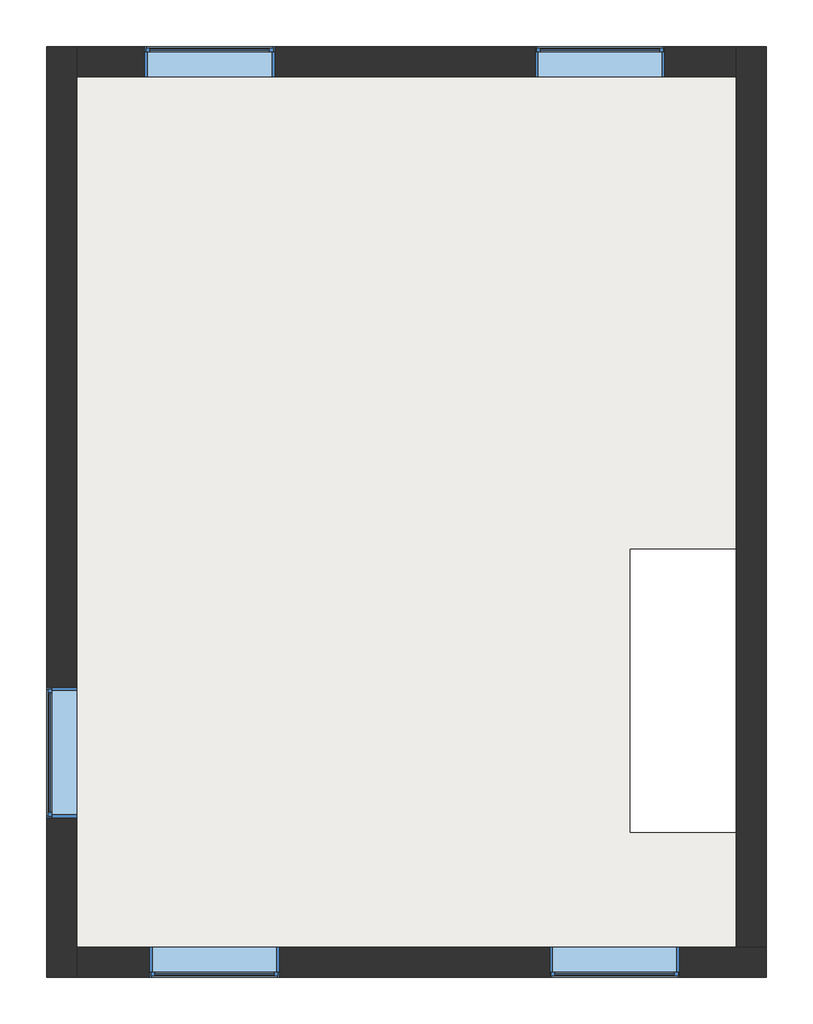
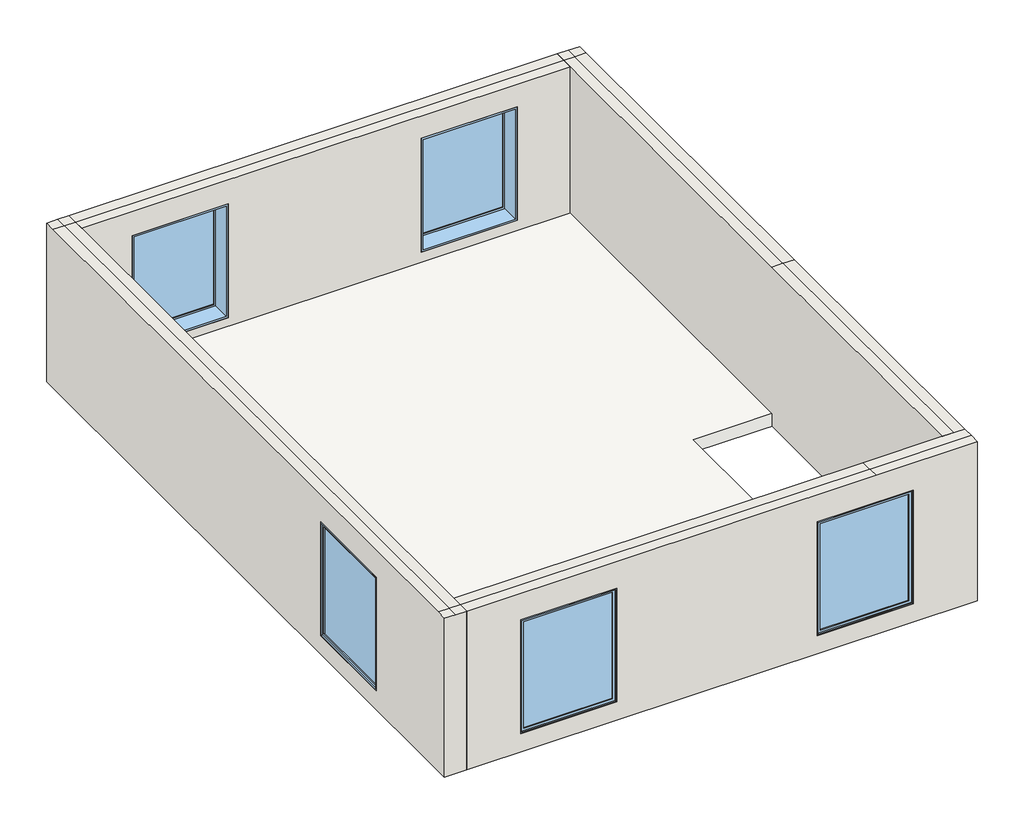
# One storey: 5 windows, 4 walls, 1 slab.
"""IFC4 building model written with IfcOpenShell, lengths in millimetres."""

import ifcopenshell
import ifcopenshell.guid

model = None  # the IFC model being written
_history = None  # IfcOwnerHistory: only IFC2X3 demands one
_inside = {}  # id of a spatial element -> (the spatial element, [elements in it])
_under = {}  # id of a project, library or spatial element -> (it, [spatial elements below it])
_declared = {}  # id of a project -> (the project, [libraries it declares])
_typed = {}  # id of a type object -> (the type object, [elements of that type])
_made_of = {}  # id of a material, layer set ... -> (it, [elements and type objects made of it])


def new_model(schema):
    """Start an empty IFC model of exactly this schema.

    Asked for "IFC4X3", IfcOpenShell would pick the latest addendum, in which some entities
    have other attributes; the version numbers below select the first issue.
    IFC2X3 requires an IfcOwnerHistory on every rooted entity: one is made here for all.
    """
    global model, _history
    if schema == "IFC4X3":
        model = ifcopenshell.file(schema_version=(4, 3, 0, 0))
    else:
        model = ifcopenshell.file(schema=schema)
    _inside.clear()
    _under.clear()
    _declared.clear()
    _typed.clear()
    _made_of.clear()
    _history = None
    if model.schema == "IFC2X3":
        org = make("IfcOrganization", Name="unknown")
        user = make(
            "IfcPersonAndOrganization",
            ThePerson=make("IfcPerson", FamilyName="unknown"),
            TheOrganization=org,
        )
        app = make(
            "IfcApplication",
            ApplicationDeveloper=org,
            Version="unknown",
            ApplicationFullName="unknown",
            ApplicationIdentifier="unknown",
        )
        _history = make(
            "IfcOwnerHistory",
            OwningUser=user,
            OwningApplication=app,
            ChangeAction="ADDED",
            CreationDate=0,
        )
    return model


def make(cls, **values):
    """One entity of the class cls with the attributes given. An attribute that is None is left unset."""
    return model.create_entity(
        cls, **{name: value for name, value in values.items() if value is not None}
    )


def rooted(cls, **values):
    """An entity with a GlobalId (a new one), such as an element, a storey or a relation."""
    return make(cls, GlobalId=ifcopenshell.guid.new(), OwnerHistory=_history, **values)


def si_unit(unit_type, name, prefix=None):
    """IfcSIUnit, for example si_unit("LENGTHUNIT", "METRE", prefix="MILLI")."""
    return make("IfcSIUnit", UnitType=unit_type, Prefix=prefix, Name=name)


def assignment(units):
    """IfcUnitAssignment: the units of a project."""
    return None if units is None else make("IfcUnitAssignment", Units=units)


def point(xyz):
    """IfcCartesianPoint."""
    return None if xyz is None else make("IfcCartesianPoint", Coordinates=xyz)


def direction(xyz):
    """IfcDirection."""
    return None if xyz is None else make("IfcDirection", DirectionRatios=xyz)


def frame(location, z_axis=None, x_axis=None):
    """IfcAxis2Placement3D, a coordinate frame: its origin and axes. An axis left out is left unset."""
    return make(
        "IfcAxis2Placement3D",
        Location=point(location),
        Axis=direction(z_axis),
        RefDirection=direction(x_axis),
    )


def origin():
    """The frame at (0, 0, 0) with its axes left unset."""
    return frame((0.0, 0.0, 0.0))


def place(relative_to, where):
    """IfcLocalPlacement: puts the frame where relative to a parent placement (None: the world)."""
    return make(
        "IfcLocalPlacement", PlacementRelTo=relative_to, RelativePlacement=where
    )


def context(
    kind, dimensions, precision=None, world=None, true_north=None, identifier=None
):
    """IfcGeometricRepresentationContext, for example the 3D "Model" context."""
    return make(
        "IfcGeometricRepresentationContext",
        ContextIdentifier=identifier,
        ContextType=kind,
        CoordinateSpaceDimension=dimensions,
        Precision=precision,
        WorldCoordinateSystem=world,
        TrueNorth=true_north,
    )


def project(units=None, contexts=None):
    """IfcProject with its units and contexts."""
    return rooted(
        "IfcProject",
        Name="project",
        RepresentationContexts=contexts,
        UnitsInContext=assignment(units),
    )


def spatial(cls, under=None, at=None, **own):
    """A site, building, storey or space (cls), placed at a placement, below another one or the project."""
    s = rooted(cls, ObjectPlacement=at, **own)
    if under is not None:
        _under.setdefault(under.id(), (under, []))[1].append(s)
    return s


def polyline(points):
    """IfcPolyline through the points."""
    return make("IfcPolyline", Points=[point(p) for p in points])


def outline(outer, holes=None, kind="AREA"):
    """IfcArbitraryClosedProfileDef: a profile drawn as a closed curve; with holes, ...WithVoids."""
    if holes is None:
        return make("IfcArbitraryClosedProfileDef", ProfileType=kind, OuterCurve=outer)
    return make(
        "IfcArbitraryProfileDefWithVoids",
        ProfileType=kind,
        OuterCurve=outer,
        InnerCurves=holes,
    )


def extrude(swept, where, along, depth):
    """IfcExtrudedAreaSolid: the profile swept, set in the frame where, extruded along a direction by depth."""
    return make(
        "IfcExtrudedAreaSolid",
        SweptArea=swept,
        Position=where,
        ExtrudedDirection=direction(along),
        Depth=depth,
    )


def faces_of(points, faces, orient=None, outer=None):
    """IfcFace entities. A face is a list of loops; a loop is a list of indices into points, from 0.

    orient and outer hold one flag for each loop. By default every Orientation is true, the
    first loop of a face is its IfcFaceOuterBound and the others are IfcFaceBound.
    """
    made = []
    for i, loops in enumerate(faces):
        bounds = []
        for j, loop in enumerate(loops):
            is_outer = j == 0 if outer is None else outer[i][j]
            bounds.append(
                make(
                    "IfcFaceOuterBound" if is_outer else "IfcFaceBound",
                    Bound=make("IfcPolyLoop", Polygon=[points[k] for k in loop]),
                    Orientation=True if orient is None else orient[i][j],
                )
            )
        made.append(make("IfcFace", Bounds=bounds))
    return made


def faceted_brep(points, faces, orient=None, outer=None, voids=None):
    """IfcFacetedBrep: a solid bounded by flat faces; with voids (closed shells), ...WithVoids."""
    shared = [point(p) for p in points]
    hull = make("IfcClosedShell", CfsFaces=faces_of(shared, faces, orient, outer))
    if voids is None:
        return make("IfcFacetedBrep", Outer=hull)
    return make(
        "IfcFacetedBrepWithVoids",
        Outer=hull,
        Voids=[
            make(cls, CfsFaces=faces_of(shared, fs, o, b)) for cls, fs, o, b in voids
        ],
    )


def shape(context_of_items, identifier, shape_type, items):
    """IfcShapeRepresentation: the items that make up one representation, for example the "Body"."""
    return make(
        "IfcShapeRepresentation",
        ContextOfItems=context_of_items,
        RepresentationIdentifier=identifier,
        RepresentationType=shape_type,
        Items=items,
    )


def source(mapping_origin, context_of_items, identifier, shape_type, items):
    """IfcRepresentationMap: a shape defined once, which mapped items show again and again."""
    return make(
        "IfcRepresentationMap",
        MappingOrigin=mapping_origin,
        MappedRepresentation=shape(context_of_items, identifier, shape_type, items),
    )


def transform(
    local_origin,
    x_axis=None,
    y_axis=None,
    z_axis=None,
    scale=None,
    scale2=None,
    scale3=None,
    uniform=True,
):
    """IfcCartesianTransformationOperator3D, or its non-uniform kind. x_axis, y_axis, z_axis: its Axis1, 2, 3."""
    if uniform:
        return make(
            "IfcCartesianTransformationOperator3D",
            Axis1=direction(x_axis),
            Axis2=direction(y_axis),
            LocalOrigin=point(local_origin),
            Scale=scale,
            Axis3=direction(z_axis),
        )
    return make(
        "IfcCartesianTransformationOperator3DnonUniform",
        Axis1=direction(x_axis),
        Axis2=direction(y_axis),
        LocalOrigin=point(local_origin),
        Scale=scale,
        Axis3=direction(z_axis),
        Scale2=scale2,
        Scale3=scale3,
    )


def mapped(mapping_source, mapping_target):
    """IfcMappedItem: shows the shape of a source again, moved by a transform."""
    return make(
        "IfcMappedItem", MappingSource=mapping_source, MappingTarget=mapping_target
    )


def made_of(thing, what):
    """Note that an element or type object is made of a material, layer set ...; save() writes the relation."""
    if what is not None:
        _made_of.setdefault(what.id(), (what, []))[1].append(thing)
    return thing


def element(
    cls,
    number,
    at=None,
    inside=None,
    cuts=None,
    type_object=None,
    material=None,
    context=None,
    identifier="Body",
    shape_type=None,
    held_by="IfcProductDefinitionShape",
    body=None,
    shapes=None,
    **own,
):
    """One element of the class cls, such as IfcWall. Its Tag is "e" and its number.

    at: its placement. inside: the storey or other place that contains it. cuts: it is an
    opening in that element (IfcRelVoidsElement). A single representation is given by context,
    identifier, shape_type and body (its items); several are given by shapes. held_by: the class
    of the entity that holds the representations. save() writes the other relations.
    """
    e = rooted(cls, Tag="e%d" % number, ObjectPlacement=at, **own)
    if body is not None:
        shapes = [shape(context, identifier, shape_type, body)]
    if shapes is not None:
        e.Representation = make(held_by, Representations=shapes)
    if inside is not None:
        _inside.setdefault(inside.id(), (inside, []))[1].append(e)
    if cuts is not None:
        rooted(
            "IfcRelVoidsElement", RelatingBuildingElement=cuts, RelatedOpeningElement=e
        )
    if type_object is not None:
        _typed.setdefault(type_object.id(), (type_object, []))[1].append(e)
    return made_of(e, material)


def aggregate(whole, parts):
    """IfcRelAggregates: a whole, such as a stair, and the parts it consists of."""
    return rooted("IfcRelAggregates", RelatingObject=whole, RelatedObjects=parts)


def save(model, path):
    """Write the relations noted so far, then the file.

    IfcRelAggregates (storeys below a building ...), IfcRelContainedInSpatialStructure (elements
    in a storey), IfcRelDefinesByType, IfcRelAssociatesMaterial and IfcRelDeclares: one each for
    every whole, place, type object, material and project.
    """
    for whole, parts in _under.values():
        aggregate(whole, parts)
    for where, things in _inside.values():
        rooted(
            "IfcRelContainedInSpatialStructure",
            RelatedElements=things,
            RelatingStructure=where,
        )
    for kind, things in _typed.values():
        rooted("IfcRelDefinesByType", RelatedObjects=things, RelatingType=kind)
    for what, things in _made_of.values():
        rooted("IfcRelAssociatesMaterial", RelatedObjects=things, RelatingMaterial=what)
    for by, libraries in _declared.values():
        rooted("IfcRelDeclares", RelatingContext=by, RelatedDefinitions=libraries)
    model.write(path)


def window_c2055f4e(model_context):
    return source(origin(), model_context, "Body", "SweptSolid", [
        extrude(outline(polyline([(-737.0, 163.0), (737.0, 163.0), (737.0, 151.0), (-737.0, 151.0), (-737.0, 163.0)])), frame((0.0, 0.0, 978.0), z_axis=(0.0, 0.0, 1.0), x_axis=(1.0, 0.0, 0.0)), (0.0, 0.0, 1.0), 1874.0),
        extrude(outline(polyline([(2896.0, -781.0), (934.0, -781.0), (934.0, 781.0), (2896.0, 781.0), (2896.0, -781.0)]), holes=[polyline([(2852.0, -737.0), (2852.0, 737.0), (978.0, 737.0), (978.0, -737.0), (2852.0, -737.0)])]), frame((0.0, 135.0, 0.0), z_axis=(0.0, 1.0, 0.0), x_axis=(0.0, 0.0, 1.0)), (0.0, 0.0, 1.0), 44.0),
        extrude(outline(polyline([(2915.0, -800.0), (915.0, -800.0), (915.0, 800.0), (2915.0, 800.0), (2915.0, -800.0)]), holes=[polyline([(2896.0, -781.0), (2896.0, 781.0), (934.0, 781.0), (934.0, -781.0), (2896.0, -781.0)])]), frame((0.0, 135.0, 0.0), z_axis=(0.0, 1.0, 0.0), x_axis=(0.0, 0.0, 1.0)), (0.0, 0.0, 1.0), 63.0),
        extrude(outline(polyline([(2915.0, -800.0), (915.0, -800.0), (915.0, 800.0), (2915.0, 800.0), (2915.0, -800.0)]), holes=[polyline([(2883.0, -768.0), (2883.0, 768.0), (947.0, 768.0), (947.0, -768.0), (2883.0, -768.0)])]), frame((0.0, -172.0, 0.0), z_axis=(0.0, 1.0, 0.0), x_axis=(0.0, 0.0, 1.0)), (0.0, 0.0, 1.0), 307.0),
    ])


model = new_model("IFC4")

# Units and contexts
model_context = context("Model", 3, world=origin())
ifc_project = project(units=[si_unit("LENGTHUNIT", "METRE", prefix="MILLI")], contexts=[model_context])

# Site, building, storey
site = spatial("IfcSite", under=ifc_project)
building = spatial("IfcBuilding", under=site)
storey = spatial("IfcBuildingStorey", under=building, Name="Уровень 3", Elevation=5600.0)

# Slab
placement = place(None, origin())
element("IfcSlab", 1, ObjectType="Монолитный бетон 225мм", at=placement, inside=storey, context=model_context, shape_type="Brep", body=[
    faceted_brep([(-10380.6631644, -2222.3774925, 5595.0), (-10380.6631644, -2222.3774925, 5820.0), (-10380.6631644, -8222.3774925, 5820.0), (-10380.6631644, -8222.3774925, 5595.0), (-11880.6631644, -13322.3774925, 5595.0), (-11880.6631644, -13322.3774925, 5820.0), (-12658.8205642, -13322.3774925, 5820.0), (-18880.6631644, -13322.3774925, 5820.0), (-18880.6631644, -13322.3774925, 5595.0), (-12658.8205642, -13322.3774925, 5595.0), (-18880.6631644, -2222.3774925, 5820.0), (-18880.6631644, -2222.3774925, 5595.0), (-10380.6631644, -13322.3774925, 5820.0), (-10380.6631644, -11722.3774925, 5820.0), (-11880.6631644, -11722.3774925, 5820.0), (-11880.6631644, -8222.3774925, 5820.0), (-11880.6631644, -8222.3774925, 5595.0), (-11880.6631644, -11722.3774925, 5595.0), (-10380.6631644, -11722.3774925, 5595.0), (-10380.6631644, -13322.3774925, 5595.0)], [[[0, 1, 2, 3]], [[4, 5, 6, 7, 8, 9]], [[8, 7, 10, 11]], [[11, 10, 1, 0]], [[10, 7, 6, 5, 12, 13, 14, 15, 2, 1]], [[11, 0, 3, 16, 17, 18, 19, 4, 9, 8]], [[3, 2, 15, 16]], [[16, 15, 14, 17]], [[17, 14, 13, 18]], [[18, 13, 12, 19]], [[19, 12, 5, 4]]]),
])

# Walls
element("IfcWall", 2, ObjectType="Типовой - Кладка 370 мм", at=placement, inside=storey, context=model_context, shape_type="Brep", body=[
    faceted_brep([(-19065.6631644, -2037.3774925, 5600.0), (-19065.6631644, -13507.3774925, 5600.0), (-19065.6631644, -13507.3774925, 8395.0), (-19065.6631644, -13322.3774925, 8395.0), (-19065.6631644, -2222.3774925, 8395.0), (-19065.6631644, -2037.3774925, 8395.0), (-19065.6631644, -11537.3774925, 5926.771933), (-19065.6631644, -9937.3774925, 5926.771933), (-19065.6631644, -9937.3774925, 7926.771933), (-19065.6631644, -11537.3774925, 7926.771933), (-18695.6631644, -2037.3774925, 5600.0), (-18695.6631644, -2037.3774925, 8395.0), (-18695.6631644, -2222.3774925, 8395.0), (-18695.6631644, -2407.3774925, 8395.0), (-18695.6631644, -13137.3774925, 8395.0), (-18695.6631644, -13322.3774925, 8395.0), (-18695.6631644, -13507.3774925, 8395.0), (-18695.6631644, -13507.3774925, 5600.0), (-18695.6631644, -13137.3774925, 5600.0), (-18695.6631644, -2407.3774925, 5600.0), (-18695.6631644, -11537.3774925, 5926.771933), (-18695.6631644, -11537.3774925, 7926.771933), (-18695.6631644, -9937.3774925, 7926.771933), (-18695.6631644, -9937.3774925, 5926.771933), (-18880.6631644, -13507.3774925, 8395.0), (-18880.6631644, -2037.3774925, 8395.0), (-18880.6631644, -2222.3774925, 8395.0), (-18880.6631644, -13322.3774925, 8395.0)], [[[0, 1, 2, 3, 4, 5], [6, 7, 8, 9]], [[10, 11, 12, 13, 14, 15, 16, 17, 18, 19], [20, 21, 22, 23]], [[1, 0, 10, 19, 18, 17]], [[2, 1, 17, 16, 24]], [[0, 5, 25, 11, 10]], [[12, 11, 25, 26]], [[5, 4, 26, 25]], [[24, 16, 15, 27]], [[4, 3, 27, 26]], [[3, 2, 24, 27]], [[15, 14, 13, 12, 26, 27]], [[21, 20, 6, 9]], [[22, 21, 9, 8]], [[23, 22, 8, 7]], [[20, 23, 7, 6]]]),
])
element("IfcWall", 3, ObjectType="Типовой - Кладка 370 мм", at=placement, inside=storey, context=model_context, shape_type="Brep", body=[
    faceted_brep([(-18695.6631644, -13507.3774925, 5600.0), (-10195.6631644, -13507.3774925, 5600.0), (-10195.6631644, -13507.3774925, 8395.0), (-11880.6631644, -13507.3774925, 8395.0), (-18695.6631644, -13507.3774925, 8395.0), (-16195.6631644, -13507.3774925, 5922.7130426), (-17795.6631644, -13507.3774925, 5922.7130426), (-17795.6631644, -13507.3774925, 7922.7130426), (-16195.6631644, -13507.3774925, 7922.7130426), (-11265.6631644, -13507.3774925, 5922.7130426), (-12865.6631644, -13507.3774925, 5922.7130426), (-12865.6631644, -13507.3774925, 7922.7130426), (-11265.6631644, -13507.3774925, 7922.7130426), (-18695.6631644, -13137.3774925, 5600.0), (-18695.6631644, -13137.3774925, 8395.0), (-11880.6631644, -13137.3774925, 8395.0), (-10565.6631644, -13137.3774925, 8395.0), (-10195.6631644, -13137.3774925, 8395.0), (-10195.6631644, -13137.3774925, 5600.0), (-10565.6631644, -13137.3774925, 5600.0), (-16195.6631644, -13137.3774925, 5922.7130426), (-16195.6631644, -13137.3774925, 7922.7130426), (-17795.6631644, -13137.3774925, 7922.7130426), (-17795.6631644, -13137.3774925, 5922.7130426), (-11265.6631644, -13137.3774925, 5922.7130426), (-11265.6631644, -13137.3774925, 7922.7130426), (-12865.6631644, -13137.3774925, 7922.7130426), (-12865.6631644, -13137.3774925, 5922.7130426), (-18695.6631644, -13322.3774925, 8395.0), (-10195.6631644, -13322.3774925, 8395.0), (-11880.6631644, -13322.3774925, 8395.0)], [[[0, 1, 2, 3, 4], [5, 6, 7, 8], [9, 10, 11, 12]], [[13, 14, 15, 16, 17, 18, 19], [20, 21, 22, 23], [24, 25, 26, 27]], [[1, 0, 13, 19, 18]], [[0, 4, 28, 14, 13]], [[2, 1, 18, 17, 29]], [[4, 3, 30, 28]], [[29, 17, 16, 15, 30]], [[3, 2, 29, 30]], [[30, 15, 14, 28]], [[21, 20, 5, 8]], [[22, 21, 8, 7]], [[23, 22, 7, 6]], [[20, 23, 6, 5]], [[25, 24, 9, 12]], [[26, 25, 12, 11]], [[27, 26, 11, 10]], [[24, 27, 10, 9]]]),
])
element("IfcWall", 4, ObjectType="Типовой - Кладка 370 мм", at=placement, inside=storey, context=model_context, shape_type="Brep", body=[
    faceted_brep([(-10195.6631644, -13137.3774925, 5600.0), (-10195.6631644, -2037.3774925, 5600.0), (-10195.6631644, -2037.3774925, 8395.0), (-10195.6631644, -2222.3774925, 8395.0), (-10195.6631644, -8222.3774925, 8395.0), (-10195.6631644, -13137.3774925, 8395.0), (-10565.6631644, -13137.3774925, 5600.0), (-10565.6631644, -13137.3774925, 8395.0), (-10565.6631644, -8222.3774925, 8395.0), (-10565.6631644, -2407.3774925, 8395.0), (-10565.6631644, -2222.3774925, 8395.0), (-10565.6631644, -2037.3774925, 8395.0), (-10565.6631644, -2037.3774925, 5600.0), (-10565.6631644, -2407.3774925, 5600.0), (-10380.6631644, -13137.3774925, 8395.0), (-10380.6631644, -2037.3774925, 8395.0), (-10380.6631644, -2222.3774925, 8395.0), (-10380.6631644, -8222.3774925, 8395.0)], [[[0, 1, 2, 3, 4, 5]], [[6, 7, 8, 9, 10, 11, 12, 13]], [[1, 0, 6, 13, 12]], [[0, 5, 14, 7, 6]], [[2, 1, 12, 11, 15]], [[15, 11, 10, 16]], [[3, 2, 15, 16]], [[8, 7, 14, 17]], [[4, 3, 16, 17]], [[5, 4, 17, 14]], [[16, 10, 9, 8, 17]]]),
])
element("IfcWall", 5, ObjectType="Типовой - Кладка 370 мм", at=placement, inside=storey, context=model_context, shape_type="Brep", body=[
    faceted_brep([(-10565.6631644, -2037.3774925, 5600.0), (-18695.6631644, -2037.3774925, 5600.0), (-18695.6631644, -2037.3774925, 8395.0), (-10565.6631644, -2037.3774925, 8395.0), (-17855.6631644, -2037.3774925, 5973.5607887), (-16255.6631644, -2037.3774925, 5973.5607887), (-16255.6631644, -2037.3774925, 7973.5607887), (-17855.6631644, -2037.3774925, 7973.5607887), (-13045.6631644, -2037.3774925, 5999.8775823), (-11445.6631644, -2037.3774925, 5999.8775823), (-11445.6631644, -2037.3774925, 7999.8775823), (-13045.6631644, -2037.3774925, 7999.8775823), (-10565.6631644, -2407.3774925, 5600.0), (-10565.6631644, -2407.3774925, 8395.0), (-18695.6631644, -2407.3774925, 8395.0), (-18695.6631644, -2407.3774925, 5600.0), (-17855.6631644, -2407.3774925, 5973.5607887), (-17855.6631644, -2407.3774925, 7973.5607887), (-16255.6631644, -2407.3774925, 7973.5607887), (-16255.6631644, -2407.3774925, 5973.5607887), (-13045.6631644, -2407.3774925, 5999.8775823), (-13045.6631644, -2407.3774925, 7999.8775823), (-11445.6631644, -2407.3774925, 7999.8775823), (-11445.6631644, -2407.3774925, 5999.8775823), (-18695.6631644, -2222.3774925, 8395.0), (-10565.6631644, -2222.3774925, 8395.0)], [[[0, 1, 2, 3], [4, 5, 6, 7], [8, 9, 10, 11]], [[12, 13, 14, 15], [16, 17, 18, 19], [20, 21, 22, 23]], [[1, 0, 12, 15]], [[2, 1, 15, 14, 24]], [[0, 3, 25, 13, 12]], [[3, 2, 24, 25]], [[24, 14, 13, 25]], [[17, 16, 4, 7]], [[18, 17, 7, 6]], [[19, 18, 6, 5]], [[16, 19, 5, 4]], [[21, 20, 8, 11]], [[22, 21, 11, 10]], [[23, 22, 10, 9]], [[20, 23, 9, 8]]]),
])

# Windows
window_shape = window_c2055f4e(model_context)
element("IfcWindow", 6, ObjectType="Фиксированные : 1600х2000", at=placement, inside=storey, context=model_context, shape_type="MappedRepresentation", body=[
    mapped(window_shape, transform((-18867.6631644, -10737.3774925, 5011.771933), x_axis=(0.0, 1.0, 0.0), y_axis=(-1.0, 0.0, 0.0), z_axis=(0.0, 0.0, 1.0))),
])
element("IfcWindow", 7, ObjectType="Фиксированные : 1600х2000", at=placement, inside=storey, context=model_context, shape_type="MappedRepresentation", body=[
    mapped(window_shape, transform((-17055.6631644, -2235.3774925, 5058.5607887), x_axis=(1.0, 0.0, 0.0), y_axis=(0.0, 1.0, 0.0), z_axis=(0.0, 0.0, 1.0))),
])
element("IfcWindow", 8, ObjectType="Фиксированные : 1600х2000", at=placement, inside=storey, context=model_context, shape_type="MappedRepresentation", body=[
    mapped(window_shape, transform((-12245.6631644, -2235.3774925, 5084.8775823), x_axis=(1.0, 0.0, 0.0), y_axis=(0.0, 1.0, 0.0), z_axis=(0.0, 0.0, 1.0))),
])
element("IfcWindow", 9, ObjectType="Фиксированные : 1600х2000", at=placement, inside=storey, context=model_context, shape_type="MappedRepresentation", body=[
    mapped(window_shape, transform((-16995.6631644, -13309.3774925, 5007.7130426), x_axis=(-1.0, 0.0, 0.0), y_axis=(0.0, -1.0, 0.0), z_axis=(0.0, 0.0, 1.0))),
])
element("IfcWindow", 10, ObjectType="Фиксированные : 1600х2000", at=placement, inside=storey, context=model_context, shape_type="MappedRepresentation", body=[
    mapped(window_shape, transform((-12065.6631644, -13309.3774925, 5007.7130426), x_axis=(-1.0, 0.0, 0.0), y_axis=(0.0, -1.0, 0.0), z_axis=(0.0, 0.0, 1.0))),
])

save(model, "model.ifc")

# Revit data of these elements
# Type "Монолитный бетон 225мм"
#   Function = 0
#   Layers, outside or top first: 50 mm "Бетон, брус для разравнивания песка/цемента" (function 1); 0 mm "Гидроизоляция" (function 100); 175 mm "Бетон, монолитный" (function 1)
# Type "Типовой - Кладка 370 мм"
#   Layers, outside or top first: 370 mm "Бетонные модули для кладки" (function 1)
# Type "Фиксированные : 1600х2000"
#   Type Mark = "20"
#   Construction Type Id = "GSP4R"
#   Analytic Construction = "Одинарное остекление стеклами Пилкингтон - 1/8 дюйма"
#   Visual Light Transmittance = 0.9
#   Solar Heat Gain Coefficient = 0.78
#   Heat Transfer Coefficient (U) = 3.6886 W/(m²·K)
#   Height = 2000 mm
#   Высота подоконника по умолчанию = 915 mm
#   Width = 1600 mm
#   Вставка окна = 19 mm
#   Наружный материал каркаса = Переплет
#   Внутренний материал каркаса = Переплет
#   Материал оконного стекла = Стекло
#   Переплет = Переплет
#   Wall Closure = (empty or 0)
# Element 1 (IfcSlab, "Монолитный бетон 225мм")
#   Height Offset From Level = 220 mm
#   built-in parameter 1001954 = 1
#   Phase Created = Новая конструкция
#   Materials on its faces: "Бетон, монолитный", "Бетон, брус для разравнивания песка/цемента"
# Elements 2, 3, 4, 5 (IfcWall, "Типовой - Кладка 370 мм")
#   Comments = ""
#   Top Offset = 0 mm
#   Base Offset = 0 mm
#   wall height = 2795 mm
#   Phase Created = Новая конструкция
#   Base Constraint = Уровень 3
#   Top Constraint = Уровень 4
#   Materials on its faces: "Бетонные модули для кладки"
# Element 6 (IfcWindow, "Фиксированные : 1600х2000")
#   Mark = "8"
#   Phase Created = Новая конструкция
#   Materials on its faces: "Переплет", "Стекло"
# Element 7 (IfcWindow, "Фиксированные : 1600х2000")
#   Mark = "9"
#   Phase Created = Новая конструкция
#   Materials on its faces: "Переплет", "Стекло"
# Element 8 (IfcWindow, "Фиксированные : 1600х2000")
#   Mark = "10"
#   Phase Created = Новая конструкция
#   Materials on its faces: "Переплет", "Стекло"
# Element 9 (IfcWindow, "Фиксированные : 1600х2000")
#   Mark = "16"
#   Phase Created = Новая конструкция
#   Materials on its faces: "Переплет", "Стекло"
# Element 10 (IfcWindow, "Фиксированные : 1600х2000")
#   Mark = "17"
#   Phase Created = Новая конструкция
#   Materials on its faces: "Переплет", "Стекло"
# Materials
#   "Бетон, брус для разравнивания песка/цемента": class "Бетон", colour RGB 127 127 127, transparency 0, Description = "Покрытие бетонной плиты", Cost = 0
#   "Гидроизоляция": class "Типовой", colour RGB 127 127 127, transparency 0, Description = "Гидроизоляция", Cost = 0
#   "Бетон, монолитный": class "Бетон", colour RGB 192 192 192, transparency 0, Description = "физический материал", Cost = 0
#   "Бетонные модули для кладки": class "Кладка", colour RGB 181 181 181, transparency 0, Description = "Бетонные модули для кладки", Cost = 0
#   "Переплет": class "Древесина", colour RGB 224 178 126, transparency 0, Cost = 0
#   "Стекло": class "Стекло", colour RGB 0 128 192, transparency 0.9, Description = "Известково-натриевое стекло", Cost = 0
